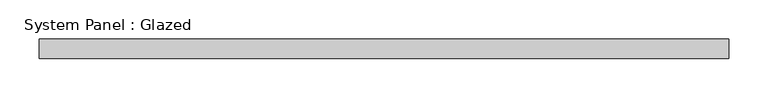
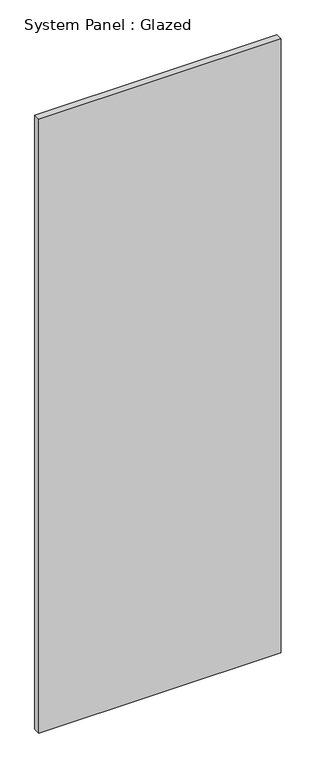
"""IFC4 building model written with IfcOpenShell, lengths in millimetres: plate geometry, System Panel : Glazed."""

from ifc_helpers import new_model, si_unit, origin, origin_with_axes, place, context, project, spatial, polyline, outline, extrude, source, transform, mapped, element, save


def system_panel_glazed_0be0c800(model_context):
    return source(origin(), model_context, "Body", "SweptSolid", [
        extrude(outline(polyline([(440.8714287, -12.7), (-440.8714287, -12.7), (-440.8714287, 12.7), (440.8714287, 12.7), (440.8714287, -12.7)])), origin_with_axes(), (0.0, 0.0, 1.0), 2362.2),
    ])


if __name__ == "__main__":
    model = new_model("IFC4")
    model_context = context("Model", 3, world=origin())
    ifc_project = project(units=[si_unit("LENGTHUNIT", "METRE", prefix="MILLI")], contexts=[model_context])
    site = spatial("IfcSite", under=ifc_project)
    building = spatial("IfcBuilding", under=site)
    placement = place(None, origin())
    system_panel_glazed_shape = system_panel_glazed_0be0c800(model_context)
    element("IfcPlate", 1, ObjectType="System Panel : Glazed", at=placement, inside=building, context=model_context, shape_type="MappedRepresentation", body=[
        mapped(system_panel_glazed_shape, transform((0.0, 0.0, 0.0), x_axis=(1.0, 0.0, 0.0), y_axis=(0.0, 1.0, 0.0), z_axis=(0.0, 0.0, 1.0))),
    ])
    save(model, "model.ifc")

# Revit data of these elements
# Element 1 (IfcPlate, "System Panel : Glazed")
#   Materials on its faces: "Glass"
# Materials
#   "Glass": class "Glass", colour RGB 218 227 224, transparency 0.85, Description = "Soda Lime Glass", Cost = 0
